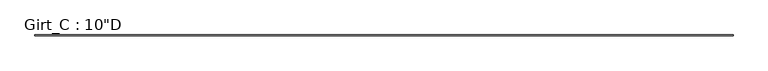
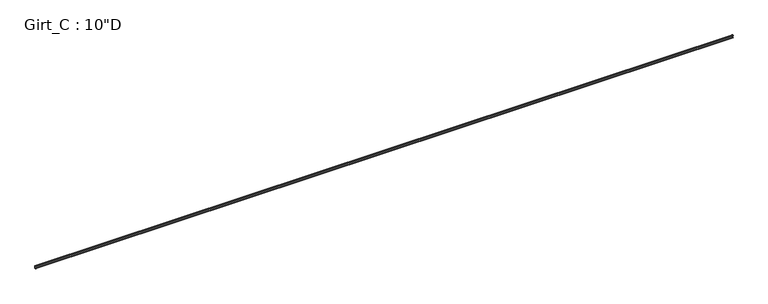
"""IFC4 building model written with IfcOpenShell, lengths in millimetres: beam geometry."""

from ifc_helpers import new_model, si_unit, point, frame, frame_2d, origin, place, context, project, spatial, polyline, circle_curve, trimmed, segment, composite_curve, outline, extrude, source, transform, mapped, element, save


def beam_8e49b336(model_context):
    return source(origin(), model_context, "Body", "SweptSolid", [
        extrude(outline(composite_curve([segment(polyline([(-87.5109375, 127.0), (-3.3734375, 127.0)]), True, "CONTINUOUS"), segment(trimmed(circle_curve(frame_2d((-3.3734375, 122.2375)), 4.7625), [point((-3.3734375, 127.0))], [point((1.3890625, 122.2375))], False, "CARTESIAN"), True, "CONTINUOUS"), segment(polyline([(1.3890625, 122.2375), (1.3890625, -122.2375)]), True, "CONTINUOUS"), segment(trimmed(circle_curve(frame_2d((-3.3734375, -122.2375)), 4.7625), [point((1.3890625, -122.2375))], [point((-3.3734375, -127.0))], False, "CARTESIAN"), True, "CONTINUOUS"), segment(polyline([(-3.3734375, -127.0), (-87.5109375, -127.0), (-99.7792647, -112.379177), (-97.6510975, -110.5934327), (-86.2154765, -124.221875), (-3.2694106, -124.221875)]), True, "CONTINUOUS"), segment(trimmed(circle_curve(frame_2d((-3.3748024, -122.2389339)), 1.9857399), [point((-3.2694106, -124.221875))], [point((-1.3890625, -122.2389339))], True, "CARTESIAN"), True, "CONTINUOUS"), segment(polyline([(-1.3890625, -122.2389339), (-1.3890625, 122.2381931)]), True, "CONTINUOUS"), segment(trimmed(circle_curve(frame_2d((-3.3741066, 122.2381931)), 1.9850441), [point((-1.3890625, 122.2381931))], [point((-3.3005807, 124.221875))], True, "CARTESIAN"), True, "CONTINUOUS"), segment(polyline([(-3.3005807, 124.221875), (-86.2154765, 124.221875), (-97.6278742, 110.621109), (-99.7560415, 112.4068534), (-87.5109375, 127.0)]), True, "CONTINUOUS")], self_intersect=False)), frame((-37433.3516, 0.0, 0.0), z_axis=(1.0, 0.0, 0.0), x_axis=(0.0, 1.0, 0.0)), (0.0, 0.0, 1.0), 74821.669),
    ])


if __name__ == "__main__":
    model = new_model("IFC4")
    model_context = context("Model", 3, world=origin())
    ifc_project = project(units=[si_unit("LENGTHUNIT", "METRE", prefix="MILLI")], contexts=[model_context])
    site = spatial("IfcSite", under=ifc_project)
    building = spatial("IfcBuilding", under=site)
    placement = place(None, origin())
    beam_shape = beam_8e49b336(model_context)
    element("IfcBeam", 1, ObjectType="Girt_C : 10\"D", at=placement, inside=building, context=model_context, shape_type="MappedRepresentation", body=[
        mapped(beam_shape, transform((0.0, 0.0, 0.0), x_axis=(1.0, 0.0, 0.0), y_axis=(0.0, 1.0, 0.0), z_axis=(0.0, 0.0, 1.0))),
    ])
    save(model, "model.ifc")

# Revit data of these elements
# Type "Girt_C : 10\"D"
#   half leg = 0' - 1 3/4"
#   Web_Thickness = 0' - 0 7/64"
#   Length [instance default] = 10' - 0"
#   Leg_1 = 0' - 3 1/2"
#   Height = 0' - 10"
#   Structural Material [instance default] = none
# Element 1 (IfcBeam, "Girt_C : 10\"D")
#   Structural Material = STRUCTURAL STEEL - SEE STRUCT. DWGS
#   Materials on its faces: "STRUCTURAL STEEL - SEE STRUCT. DWGS"
# Materials
#   "STRUCTURAL STEEL - SEE STRUCT. DWGS": class "Metal", colour RGB 137 146 153, transparency 0, Description = "Steel, mill finish", Cost = 0
